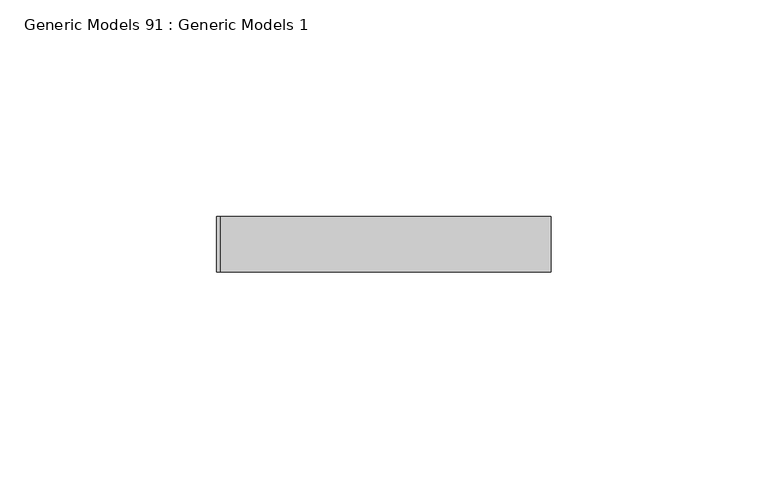
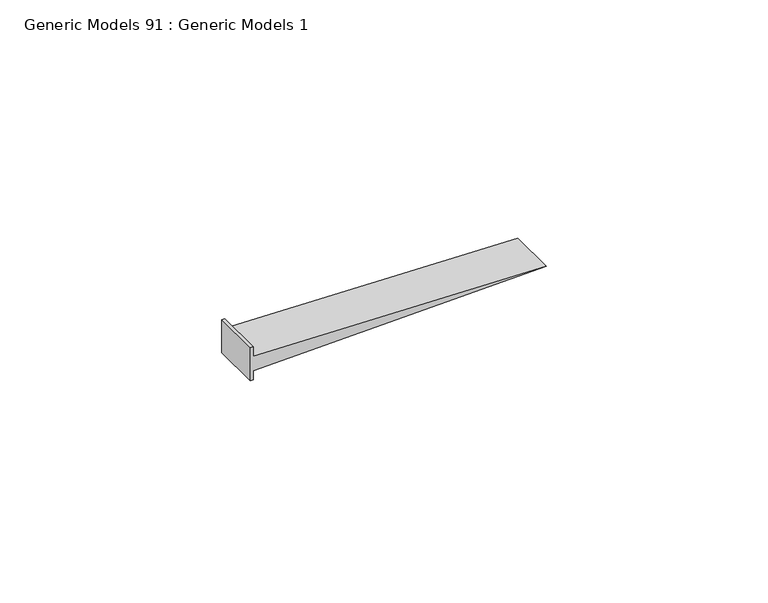
"""IFC4 building model written with IfcOpenShell, lengths in millimetres: proxy geometry, Generic Models 91 : Generic Models 1."""

from ifc_helpers import new_model, si_unit, frame, origin, place, context, project, spatial, polyline, outline, extrude, source, transform, mapped, element, save


def generic_models_91_generic_models_1_b13b52c1(model_context):
    return source(origin(), model_context, "Body", "SweptSolid", [
        extrude(outline(polyline([(2442.2225782, 49675.25625), (2433.1293782, 49675.25625), (2433.1293782, 49676.05), (2435.6792418, 49676.05), (2437.6759782, 49752.25), (2439.6727146, 49676.05), (2442.2225782, 49676.05), (2442.2225782, 49675.25625)])), frame((0.0, 565.15, 0.0), z_axis=(0.0, 1.0, 0.0), x_axis=(0.0, 0.0, 1.0)), (0.0, 0.0, 1.0), 12.7),
    ])


if __name__ == "__main__":
    model = new_model("IFC4")
    model_context = context("Model", 3, world=origin())
    ifc_project = project(units=[si_unit("LENGTHUNIT", "METRE", prefix="MILLI")], contexts=[model_context])
    site = spatial("IfcSite", under=ifc_project)
    building = spatial("IfcBuilding", under=site)
    placement = place(None, origin())
    generic_models_91_generic_models_1_shape = generic_models_91_generic_models_1_b13b52c1(model_context)
    element("IfcBuildingElementProxy", 1, Name="Generic Models 91 : Generic Models 1", ObjectType="Generic Models 91 : Generic Models 1", at=placement, inside=building, context=model_context, shape_type="MappedRepresentation", body=[
        mapped(generic_models_91_generic_models_1_shape, transform((0.0, 0.0, 0.0), x_axis=(1.0, 0.0, 0.0), y_axis=(0.0, 1.0, 0.0), z_axis=(0.0, 0.0, 1.0))),
    ])
    save(model, "model.ifc")

# Revit data of these elements
# Element 1 (IfcBuildingElementProxy, "Generic Models 91 : Generic Models 1")
#   Materials on its faces: "ATTACH GYPSUM BOARD TO STUDS AND NOT TO TOP TRACK"
# Materials
#   "ATTACH GYPSUM BOARD TO STUDS AND NOT TO TOP TRACK": class "Generic", colour RGB 48 48 48, transparency 0, Cost = 0
